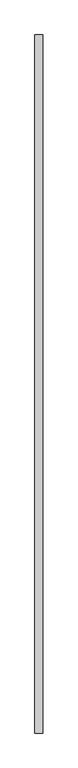
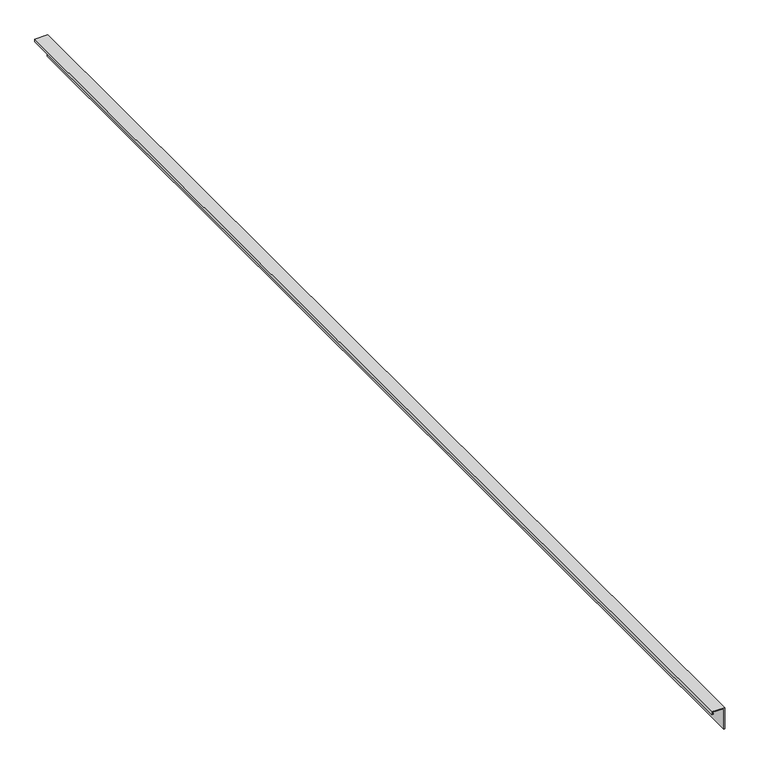
"""IFC4 building model written with IfcOpenShell, lengths in millimetres: proxy geometry, GRAVEL STOP17:GRAVEL STOP003:306582 : GRAVEL STOP17:GRAVEL STOP003:306582."""

from ifc_helpers import new_model, si_unit, frame, origin, place, context, project, spatial, polyline, outline, extrude, source, transform, mapped, element, save


def generic_models_5f688081(model_context):
    return source(origin(), model_context, "Body", "SweptSolid", [
        extrude(outline(polyline([(40234.4061757, 1966.5954611), (40234.4061757, 1986.2804611), (40197.5761757, 1986.2804611), (40197.5761757, 1987.5504611), (40235.6761757, 1987.5504611), (40235.6761757, 1965.3254611), (40230.9263757, 1965.3254611), (40230.9263757, 1968.3279174), (40232.1963757, 1968.3279174), (40232.1963757, 1966.5954611), (40234.4061757, 1966.5954611)])), frame((0.0, -774.5581162, 0.0), z_axis=(0.0, 1.0, 0.0), x_axis=(0.0, 0.0, 1.0)), (0.0, 0.0, 1.0), 2000.25),
    ])


if __name__ == "__main__":
    model = new_model("IFC4")
    model_context = context("Model", 3, world=origin())
    ifc_project = project(units=[si_unit("LENGTHUNIT", "METRE", prefix="MILLI")], contexts=[model_context])
    site = spatial("IfcSite", under=ifc_project)
    building = spatial("IfcBuilding", under=site)
    placement = place(None, origin())
    generic_models_shape = generic_models_5f688081(model_context)
    element("IfcBuildingElementProxy", 1, Name="GRAVEL STOP17:GRAVEL STOP003:306582 : GRAVEL STOP17:GRAVEL STOP003:306582", ObjectType="GRAVEL STOP17:GRAVEL STOP003:306582 : GRAVEL STOP17:GRAVEL STOP003:306582", at=placement, inside=building, context=model_context, shape_type="MappedRepresentation", body=[
        mapped(generic_models_shape, transform((0.0, 0.0, 0.0), x_axis=(1.0, 0.0, 0.0), y_axis=(0.0, 1.0, 0.0), z_axis=(0.0, 0.0, 1.0))),
    ])
    save(model, "model.ifc")

# Revit data of these elements
# Type "GRAVEL STOP17:GRAVEL STOP003:306582 : GRAVEL STOP17:GRAVEL STOP003:306582"
#   NameOverride = "GRAVEL STOP17:GRAVEL STOP003:306582"
#   ObjectTypeOverride = "GRAVEL STOP17:GRAVEL STOP003"
#   Reference = "GRAVEL STOP003"
#   Category = "Generic Models"
#   Tag = "306582"
# Element 1 (IfcBuildingElementProxy, "GRAVEL STOP17:GRAVEL STOP003:306582 : GRAVEL STOP17:GRAVEL STOP003:306582")
#   Materials on its faces: "COPPER STUCCO J BEAD"
# Materials
#   "COPPER STUCCO J BEAD": class "Unassigned", colour RGB 251 232 155, transparency 0, Cost = 0
